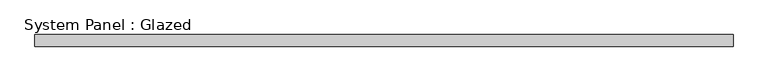
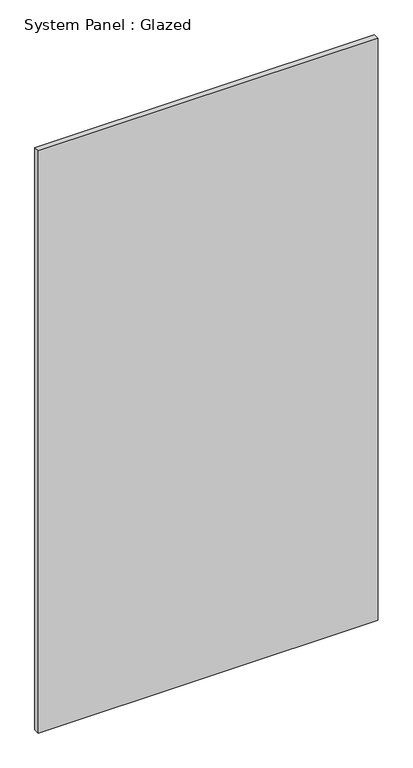
"""IFC4 building model written with IfcOpenShell, lengths in millimetres: plate geometry, System Panel : Glazed."""

from ifc_helpers import new_model, si_unit, origin, origin_with_axes, place, context, project, spatial, polyline, outline, extrude, source, transform, mapped, element, save


def system_panel_glazed_ab17d442(model_context):
    return source(origin(), model_context, "Body", "SweptSolid", [
        extrude(outline(polyline([(724.9999999, 24.5), (-724.9999999, 24.5), (-724.9999999, 49.5), (724.9999999, 49.5), (724.9999999, 24.5)])), origin_with_axes(), (0.0, 0.0, 1.0), 2625.0),
    ])


if __name__ == "__main__":
    model = new_model("IFC4")
    model_context = context("Model", 3, world=origin())
    ifc_project = project(units=[si_unit("LENGTHUNIT", "METRE", prefix="MILLI")], contexts=[model_context])
    site = spatial("IfcSite", under=ifc_project)
    building = spatial("IfcBuilding", under=site)
    placement = place(None, origin())
    system_panel_glazed_shape = system_panel_glazed_ab17d442(model_context)
    element("IfcPlate", 1, ObjectType="System Panel : Glazed", at=placement, inside=building, context=model_context, shape_type="MappedRepresentation", body=[
        mapped(system_panel_glazed_shape, transform((0.0, 0.0, 0.0), x_axis=(1.0, 0.0, 0.0), y_axis=(0.0, 1.0, 0.0), z_axis=(0.0, 0.0, 1.0))),
    ])
    save(model, "model.ifc")

# Revit data of these elements
# Type "System Panel : Glazed"
#   Keynote = "H11"
#   Construction Type Id = "GSP4R"
#   Analytic Construction = "1/8 in Pilkington single glazing"
#   Visual Light Transmittance = 0.9
#   Solar Heat Gain Coefficient = 0.86
#   Heat Transfer Coefficient (U) = 6.7069 W/(m²·K)
# Element 1 (IfcPlate, "System Panel : Glazed")
#   Materials on its faces: "Glass"
# Materials
#   "Glass": class "Glass", colour RGB 0 128 192, transparency 0.9, Description = "Soda Lime Glass", Cost = 0
